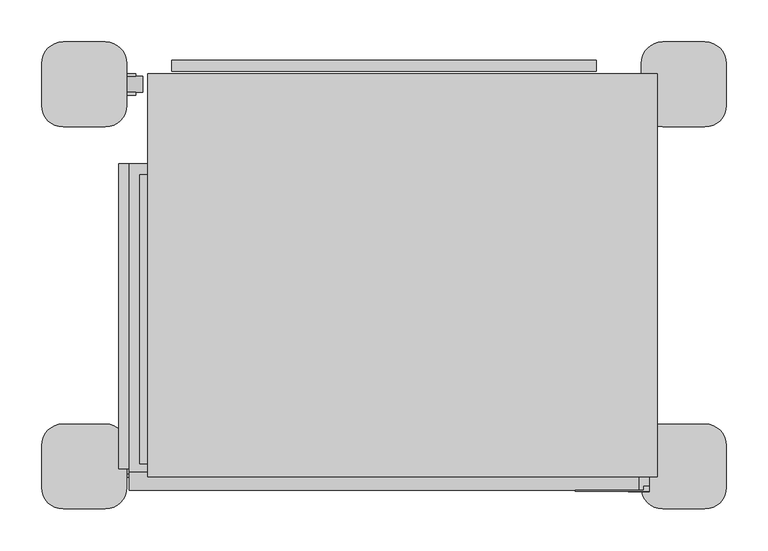
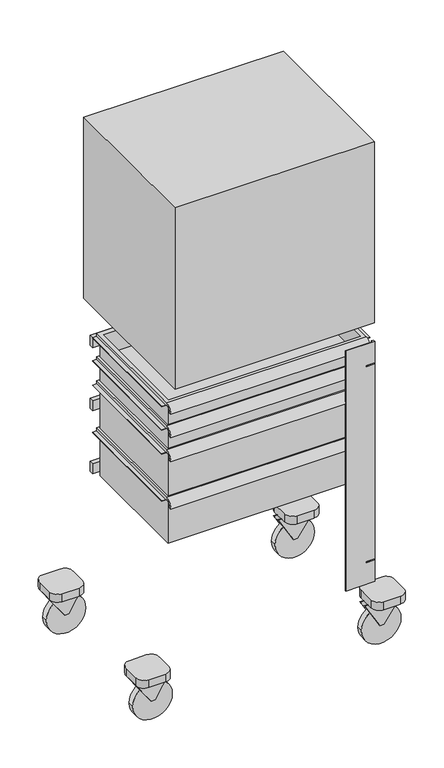
"""IFC4 building model written with IfcOpenShell, lengths in millimetres: proxy geometry, M8185 - System, Stress Exercise, w-Treadmill : M8185 - System, Stress Exercise, w-Treadmill."""

import ifcopenshell
import ifcopenshell.guid

model = None  # the IFC model being written
_history = None  # IfcOwnerHistory: only IFC2X3 demands one
_inside = {}  # id of a spatial element -> (the spatial element, [elements in it])
_under = {}  # id of a project, library or spatial element -> (it, [spatial elements below it])
_declared = {}  # id of a project -> (the project, [libraries it declares])
_typed = {}  # id of a type object -> (the type object, [elements of that type])
_made_of = {}  # id of a material, layer set ... -> (it, [elements and type objects made of it])


def new_model(schema):
    """Start an empty IFC model of exactly this schema.

    Asked for "IFC4X3", IfcOpenShell would pick the latest addendum, in which some entities
    have other attributes; the version numbers below select the first issue.
    IFC2X3 requires an IfcOwnerHistory on every rooted entity: one is made here for all.
    """
    global model, _history
    if schema == "IFC4X3":
        model = ifcopenshell.file(schema_version=(4, 3, 0, 0))
    else:
        model = ifcopenshell.file(schema=schema)
    _inside.clear()
    _under.clear()
    _declared.clear()
    _typed.clear()
    _made_of.clear()
    _history = None
    if model.schema == "IFC2X3":
        org = make("IfcOrganization", Name="unknown")
        user = make(
            "IfcPersonAndOrganization",
            ThePerson=make("IfcPerson", FamilyName="unknown"),
            TheOrganization=org,
        )
        app = make(
            "IfcApplication",
            ApplicationDeveloper=org,
            Version="unknown",
            ApplicationFullName="unknown",
            ApplicationIdentifier="unknown",
        )
        _history = make(
            "IfcOwnerHistory",
            OwningUser=user,
            OwningApplication=app,
            ChangeAction="ADDED",
            CreationDate=0,
        )
    return model


def make(cls, **values):
    """One entity of the class cls with the attributes given. An attribute that is None is left unset."""
    return model.create_entity(
        cls, **{name: value for name, value in values.items() if value is not None}
    )


def rooted(cls, **values):
    """An entity with a GlobalId (a new one), such as an element, a storey or a relation."""
    return make(cls, GlobalId=ifcopenshell.guid.new(), OwnerHistory=_history, **values)


def si_unit(unit_type, name, prefix=None):
    """IfcSIUnit, for example si_unit("LENGTHUNIT", "METRE", prefix="MILLI")."""
    return make("IfcSIUnit", UnitType=unit_type, Prefix=prefix, Name=name)


def assignment(units):
    """IfcUnitAssignment: the units of a project."""
    return None if units is None else make("IfcUnitAssignment", Units=units)


def point(xyz):
    """IfcCartesianPoint."""
    return None if xyz is None else make("IfcCartesianPoint", Coordinates=xyz)


def direction(xyz):
    """IfcDirection."""
    return None if xyz is None else make("IfcDirection", DirectionRatios=xyz)


def frame(location, z_axis=None, x_axis=None):
    """IfcAxis2Placement3D, a coordinate frame: its origin and axes. An axis left out is left unset."""
    return make(
        "IfcAxis2Placement3D",
        Location=point(location),
        Axis=direction(z_axis),
        RefDirection=direction(x_axis),
    )


def frame_2d(location, x_axis=None):
    """IfcAxis2Placement2D, a coordinate frame in the plane: its origin and x axis."""
    return make(
        "IfcAxis2Placement2D", Location=point(location), RefDirection=direction(x_axis)
    )


def origin():
    """The frame at (0, 0, 0) with its axes left unset."""
    return frame((0.0, 0.0, 0.0))


def place(relative_to, where):
    """IfcLocalPlacement: puts the frame where relative to a parent placement (None: the world)."""
    return make(
        "IfcLocalPlacement", PlacementRelTo=relative_to, RelativePlacement=where
    )


def context(
    kind, dimensions, precision=None, world=None, true_north=None, identifier=None
):
    """IfcGeometricRepresentationContext, for example the 3D "Model" context."""
    return make(
        "IfcGeometricRepresentationContext",
        ContextIdentifier=identifier,
        ContextType=kind,
        CoordinateSpaceDimension=dimensions,
        Precision=precision,
        WorldCoordinateSystem=world,
        TrueNorth=true_north,
    )


def project(units=None, contexts=None):
    """IfcProject with its units and contexts."""
    return rooted(
        "IfcProject",
        Name="project",
        RepresentationContexts=contexts,
        UnitsInContext=assignment(units),
    )


def spatial(cls, under=None, at=None, **own):
    """A site, building, storey or space (cls), placed at a placement, below another one or the project."""
    s = rooted(cls, ObjectPlacement=at, **own)
    if under is not None:
        _under.setdefault(under.id(), (under, []))[1].append(s)
    return s


def polyline(points):
    """IfcPolyline through the points."""
    return make("IfcPolyline", Points=[point(p) for p in points])


def circle_curve(where, radius):
    """IfcCircle in the frame where."""
    return make("IfcCircle", Position=where, Radius=radius)


def trimmed(basis, trim1, trim2, sense, master):
    """IfcTrimmedCurve: the piece of a basis curve between two trims."""
    return make(
        "IfcTrimmedCurve",
        BasisCurve=basis,
        Trim1=trim1,
        Trim2=trim2,
        SenseAgreement=sense,
        MasterRepresentation=master,
    )


def segment(curve, same_sense, transition):
    """IfcCompositeCurveSegment."""
    return make(
        "IfcCompositeCurveSegment",
        Transition=transition,
        SameSense=same_sense,
        ParentCurve=curve,
    )


def composite_curve(segments, self_intersect=None):
    """IfcCompositeCurve: segments joined end to end."""
    return make("IfcCompositeCurve", Segments=segments, SelfIntersect=self_intersect)


def outline(outer, holes=None, kind="AREA"):
    """IfcArbitraryClosedProfileDef: a profile drawn as a closed curve; with holes, ...WithVoids."""
    if holes is None:
        return make("IfcArbitraryClosedProfileDef", ProfileType=kind, OuterCurve=outer)
    return make(
        "IfcArbitraryProfileDefWithVoids",
        ProfileType=kind,
        OuterCurve=outer,
        InnerCurves=holes,
    )


def extrude(swept, where, along, depth):
    """IfcExtrudedAreaSolid: the profile swept, set in the frame where, extruded along a direction by depth."""
    return make(
        "IfcExtrudedAreaSolid",
        SweptArea=swept,
        Position=where,
        ExtrudedDirection=direction(along),
        Depth=depth,
    )


def faces_of(points, faces, orient=None, outer=None):
    """IfcFace entities. A face is a list of loops; a loop is a list of indices into points, from 0.

    orient and outer hold one flag for each loop. By default every Orientation is true, the
    first loop of a face is its IfcFaceOuterBound and the others are IfcFaceBound.
    """
    made = []
    for i, loops in enumerate(faces):
        bounds = []
        for j, loop in enumerate(loops):
            is_outer = j == 0 if outer is None else outer[i][j]
            bounds.append(
                make(
                    "IfcFaceOuterBound" if is_outer else "IfcFaceBound",
                    Bound=make("IfcPolyLoop", Polygon=[points[k] for k in loop]),
                    Orientation=True if orient is None else orient[i][j],
                )
            )
        made.append(make("IfcFace", Bounds=bounds))
    return made


def faceted_brep(points, faces, orient=None, outer=None, voids=None):
    """IfcFacetedBrep: a solid bounded by flat faces; with voids (closed shells), ...WithVoids."""
    shared = [point(p) for p in points]
    hull = make("IfcClosedShell", CfsFaces=faces_of(shared, faces, orient, outer))
    if voids is None:
        return make("IfcFacetedBrep", Outer=hull)
    return make(
        "IfcFacetedBrepWithVoids",
        Outer=hull,
        Voids=[
            make(cls, CfsFaces=faces_of(shared, fs, o, b)) for cls, fs, o, b in voids
        ],
    )


def shape(context_of_items, identifier, shape_type, items):
    """IfcShapeRepresentation: the items that make up one representation, for example the "Body"."""
    return make(
        "IfcShapeRepresentation",
        ContextOfItems=context_of_items,
        RepresentationIdentifier=identifier,
        RepresentationType=shape_type,
        Items=items,
    )


def source(mapping_origin, context_of_items, identifier, shape_type, items):
    """IfcRepresentationMap: a shape defined once, which mapped items show again and again."""
    return make(
        "IfcRepresentationMap",
        MappingOrigin=mapping_origin,
        MappedRepresentation=shape(context_of_items, identifier, shape_type, items),
    )


def transform(
    local_origin,
    x_axis=None,
    y_axis=None,
    z_axis=None,
    scale=None,
    scale2=None,
    scale3=None,
    uniform=True,
):
    """IfcCartesianTransformationOperator3D, or its non-uniform kind. x_axis, y_axis, z_axis: its Axis1, 2, 3."""
    if uniform:
        return make(
            "IfcCartesianTransformationOperator3D",
            Axis1=direction(x_axis),
            Axis2=direction(y_axis),
            LocalOrigin=point(local_origin),
            Scale=scale,
            Axis3=direction(z_axis),
        )
    return make(
        "IfcCartesianTransformationOperator3DnonUniform",
        Axis1=direction(x_axis),
        Axis2=direction(y_axis),
        LocalOrigin=point(local_origin),
        Scale=scale,
        Axis3=direction(z_axis),
        Scale2=scale2,
        Scale3=scale3,
    )


def mapped(mapping_source, mapping_target):
    """IfcMappedItem: shows the shape of a source again, moved by a transform."""
    return make(
        "IfcMappedItem", MappingSource=mapping_source, MappingTarget=mapping_target
    )


def made_of(thing, what):
    """Note that an element or type object is made of a material, layer set ...; save() writes the relation."""
    if what is not None:
        _made_of.setdefault(what.id(), (what, []))[1].append(thing)
    return thing


def element(
    cls,
    number,
    at=None,
    inside=None,
    cuts=None,
    type_object=None,
    material=None,
    context=None,
    identifier="Body",
    shape_type=None,
    held_by="IfcProductDefinitionShape",
    body=None,
    shapes=None,
    **own,
):
    """One element of the class cls, such as IfcWall. Its Tag is "e" and its number.

    at: its placement. inside: the storey or other place that contains it. cuts: it is an
    opening in that element (IfcRelVoidsElement). A single representation is given by context,
    identifier, shape_type and body (its items); several are given by shapes. held_by: the class
    of the entity that holds the representations. save() writes the other relations.
    """
    e = rooted(cls, Tag="e%d" % number, ObjectPlacement=at, **own)
    if body is not None:
        shapes = [shape(context, identifier, shape_type, body)]
    if shapes is not None:
        e.Representation = make(held_by, Representations=shapes)
    if inside is not None:
        _inside.setdefault(inside.id(), (inside, []))[1].append(e)
    if cuts is not None:
        rooted(
            "IfcRelVoidsElement", RelatingBuildingElement=cuts, RelatedOpeningElement=e
        )
    if type_object is not None:
        _typed.setdefault(type_object.id(), (type_object, []))[1].append(e)
    return made_of(e, material)


def aggregate(whole, parts):
    """IfcRelAggregates: a whole, such as a stair, and the parts it consists of."""
    return rooted("IfcRelAggregates", RelatingObject=whole, RelatedObjects=parts)


def save(model, path):
    """Write the relations noted so far, then the file.

    IfcRelAggregates (storeys below a building ...), IfcRelContainedInSpatialStructure (elements
    in a storey), IfcRelDefinesByType, IfcRelAssociatesMaterial and IfcRelDeclares: one each for
    every whole, place, type object, material and project.
    """
    for whole, parts in _under.values():
        aggregate(whole, parts)
    for where, things in _inside.values():
        rooted(
            "IfcRelContainedInSpatialStructure",
            RelatedElements=things,
            RelatingStructure=where,
        )
    for kind, things in _typed.values():
        rooted("IfcRelDefinesByType", RelatedObjects=things, RelatingType=kind)
    for what, things in _made_of.values():
        rooted("IfcRelAssociatesMaterial", RelatedObjects=things, RelatingMaterial=what)
    for by, libraries in _declared.values():
        rooted("IfcRelDeclares", RelatingContext=by, RelatedDefinitions=libraries)
    model.write(path)


def plane_surface(at):
    """IfcPlane: the flat surface through the origin of the frame at, square to its z axis."""
    return make("IfcPlane", Position=at)


def cylinder_surface(at, radius):
    """IfcCylindricalSurface: all points at the distance radius from the z axis of the frame at."""
    return make("IfcCylindricalSurface", Position=at, Radius=radius)


def revolved_surface(curve, axis_point, axis_direction):
    """IfcSurfaceOfRevolution: the curve turned about the line through axis_point along axis_direction."""
    return make(
        "IfcSurfaceOfRevolution",
        SweptCurve=make("IfcArbitraryOpenProfileDef", ProfileType="CURVE", Curve=curve),
        AxisPosition=make("IfcAxis1Placement", Location=point(axis_point), Axis=direction(axis_direction)),
    )


def advanced_brep(points, edges, surfaces, faces):
    """IfcAdvancedBrep: a solid bounded by faces that lie on surfaces and meet in shared edges.

    An edge is (start, end): straight between two places in points (the first is 0);
    or (start, end, curve); or (start, end, curve, False) where it runs against its curve.
    A face is (place in surfaces, loops), or (place, loops, False) where it looks against
    its surface's normal. A loop lists edges by number (the first is 1), with a minus sign
    where the edge is run from its end to its start. The first loop is the outer one.
    """
    corners = [point(p) for p in points]
    vertices = [make("IfcVertexPoint", VertexGeometry=c) for c in corners]
    made = []
    for start, end, *more in edges:
        made.append(
            make(
                "IfcEdgeCurve",
                EdgeStart=vertices[start],
                EdgeEnd=vertices[end],
                EdgeGeometry=more[0] if more else make("IfcPolyline", Points=[corners[start], corners[end]]),
                SameSense=more[1] if len(more) > 1 else True,
            )
        )
    hull = []
    for where, loops, *sense in faces:
        bounds = []
        for j, loop in enumerate(loops):
            ring = [make("IfcOrientedEdge", EdgeElement=made[abs(k) - 1], Orientation=k > 0) for k in loop]
            bounds.append(
                make(
                    "IfcFaceOuterBound" if j == 0 else "IfcFaceBound",
                    Bound=make("IfcEdgeLoop", EdgeList=ring),
                    Orientation=True,
                )
            )
        hull.append(make("IfcAdvancedFace", Bounds=bounds, FaceSurface=surfaces[where], SameSense=sense[0] if sense else True))
    return make("IfcAdvancedBrep", Outer=make("IfcClosedShell", CfsFaces=hull))


def specialty_equipment_8ec998c3(model_context):
    return source(origin(), model_context, "Body", "SolidModel", [
        faceted_brep([(-177.3747223, 933.9418342, 1473.2), (-659.9747223, 933.9418342, 1473.2), (-659.9747223, 883.3104531, 1473.2), (-177.3747223, 883.3104531, 1473.2), (-177.3747223, 933.9418342, 1193.8), (-177.3747223, 883.3104531, 1193.8), (-659.9747223, 883.3104531, 1193.8), (-659.9747223, 933.9418342, 1193.8), (-647.2747223, 883.3104531, 1460.5), (-190.0747223, 883.3104531, 1460.5), (-190.0747223, 883.3104531, 1206.5), (-647.2747223, 883.3104531, 1206.5), (-190.0747223, 888.0966556, 1460.5), (-647.2747223, 888.0966556, 1460.5), (-190.0747223, 888.0966556, 1206.5), (-647.2747223, 888.0966556, 1206.5)], [[[0, 1, 2, 3]], [[4, 5, 6, 7]], [[1, 0, 4, 7]], [[2, 1, 7, 6]], [[3, 2, 6, 5], [8, 9, 10, 11]], [[0, 3, 5, 4]], [[12, 9, 8, 13]], [[14, 15, 11, 10]], [[12, 13, 15, 14]], [[13, 8, 11, 15]], [[9, 12, 14, 10]]]),
        extrude(outline(polyline([(584.7761437, 1054.1), (737.1761437, 1066.8), (737.1761437, 1041.4), (584.7761437, 1041.4), (584.7761437, 1054.1)])), frame((-659.9747223, 0.0, 0.0), z_axis=(1.0, 0.0, 0.0), x_axis=(0.0, 1.0, 0.0)), (0.0, 0.0, 1.0), 482.6),
        faceted_brep([(-271.4528828, 800.6761437, 1066.8), (-271.4528828, 800.6761437, 1041.4), (-271.4528828, 1016.5761437, 1041.4), (-271.4528828, 1016.5761437, 1066.8), (-565.8965618, 1016.5761437, 1066.8), (-565.8965618, 1016.5761437, 1041.4), (-565.8965618, 800.6761437, 1041.4), (-565.8965618, 800.6761437, 1066.8), (-381.7061537, 997.4418342, 1073.15), (-381.7061537, 997.4418342, 1066.8), (-455.6432909, 997.4418342, 1066.8), (-455.6432909, 997.4418342, 1073.15), (-381.7061537, 997.4418342, 1333.5), (-455.6432909, 997.4418342, 1333.5), (-381.7061537, 933.9418342, 1333.5), (-455.6432909, 933.9418342, 1333.5), (-381.7061537, 933.9418342, 1282.7), (-455.6432909, 933.9418342, 1282.7), (-381.7061537, 972.0418342, 1282.7), (-455.6432909, 972.0418342, 1282.7), (-381.7061537, 972.0418342, 1066.8), (-455.6432909, 972.0418342, 1066.8)], [[[0, 1, 2, 3]], [[4, 5, 6, 7]], [[8, 9, 10, 11]], [[12, 8, 11, 13]], [[14, 12, 13, 15]], [[16, 14, 15, 17]], [[18, 16, 17, 19]], [[20, 18, 19, 21]], [[0, 3, 4, 7], [9, 20, 21, 10]], [[1, 0, 7, 6]], [[2, 1, 6, 5]], [[3, 2, 5, 4]], [[20, 9, 8, 12, 14, 16, 18]], [[10, 21, 19, 17, 15, 13, 11]]]),
        extrude(outline(polyline([(-113.8747223, 1041.9761437), (-113.8747223, 559.3761437), (-723.4747223, 559.3761437), (-723.4747223, 1041.9761437), (-113.8747223, 1041.9761437)])), frame((0.0, 0.0, 1041.4), z_axis=(0.0, 0.0, 1.0), x_axis=(1.0, 0.0, 0.0)), (0.0, 0.0, 1.0), 584.2),
        extrude(outline(polyline([(-186.8997223, 1057.8511437), (-186.8997223, 1045.1511437), (-694.8997223, 1045.1511437), (-694.8997223, 1057.8511437), (-186.8997223, 1057.8511437)])), frame((0.0, 0.0, 464.30692), z_axis=(0.0, 0.0, 1.0), x_axis=(1.0, 0.0, 0.0)), (0.0, 0.0, 1.0), 31.75),
        extrude(outline(polyline([(-186.8997223, 1057.8511437), (-186.8997223, 1045.1511437), (-694.8997223, 1045.1511437), (-694.8997223, 1057.8511437), (-186.8997223, 1057.8511437)])), frame((0.0, 0.0, 667.50692), z_axis=(0.0, 0.0, 1.0), x_axis=(1.0, 0.0, 0.0)), (0.0, 0.0, 1.0), 31.75),
        extrude(outline(polyline([(-186.8997223, 1057.8511437), (-186.8997223, 1045.1511437), (-694.8997223, 1045.1511437), (-694.8997223, 1057.8511437), (-186.8997223, 1057.8511437)])), frame((0.0, 0.0, 870.70692), z_axis=(0.0, 0.0, 1.0), x_axis=(1.0, 0.0, 0.0)), (0.0, 0.0, 1.0), 31.75),
        advanced_brep(
        [(-739.3497223, 569.0376764, 696.8915302), (-142.4497223, 569.0376764, 696.8915302), (-142.4497223, 569.0376764, 838.1917302), (-123.3997223, 569.0376764, 838.1917302), (-123.3997223, 569.0376764, 839.7792302), (-136.0997223, 569.0376764, 839.7792302), (-136.0997223, 569.0376764, 842.9415302), (-745.6997223, 569.0376764, 842.9415302), (-745.6997223, 569.0376764, 839.7792302), (-758.3997223, 569.0376764, 839.7792302), (-758.3997223, 569.0376764, 838.1917302), (-739.3497223, 569.0376764, 838.1917302), (-142.4497223, 927.8126764, 696.8915302), (-739.3497223, 927.8126764, 696.8915302), (-739.3497223, 927.8126764, 838.1917302), (-142.4497223, 927.8126764, 838.1917302), (-136.0997223, 565.7634577, 849.2915302), (-136.0997223, 934.1626764, 849.2915302), (-745.6997223, 934.1626764, 849.2915302), (-745.6997223, 565.7634577, 849.2915302), (-148.7997223, 575.3876764, 849.2915302), (-732.9997223, 575.3876764, 849.2915302), (-732.9997223, 920.8276764, 849.2915302), (-148.7997223, 920.8276764, 849.2915302), (-136.0997223, 543.6376764, 824.6484502), (-136.0997223, 550.0395136, 824.6484502), (-136.0997223, 565.7634577, 842.9415302), (-136.0997223, 934.1626764, 839.7792302), (-745.6997223, 565.7634577, 842.9415302), (-745.6997223, 550.0395136, 824.6484502), (-745.6997223, 543.6376764, 824.6484502), (-745.6997223, 934.1626764, 839.7792302), (-123.3997223, 934.1626764, 838.1917302), (-758.3997223, 934.1626764, 838.1917302), (-123.3997223, 934.1626764, 839.7792302), (-758.3997223, 934.1626764, 839.7792302), (-732.9997223, 575.3876764, 706.4165302), (-148.7997223, 575.3876764, 706.4165302), (-148.7997223, 920.8276764, 706.4165302), (-732.9997223, 920.8276764, 706.4165302)],
        [
            (0, 1),
            (1, 2),
            (2, 3),
            (3, 4),
            (4, 5),
            (5, 6),
            (6, 7),
            (7, 8),
            (8, 9),
            (9, 10),
            (10, 11),
            (11, 0),
            (12, 13),
            (13, 14),
            (14, 15),
            (15, 12),
            (0, 13),
            (12, 1),
            (15, 2),
            (16, 17),
            (17, 18),
            (18, 19),
            (19, 16),
            (20, 21),
            (21, 22),
            (22, 23),
            (23, 20),
            (11, 14),
            (16, 24, circle_curve(frame((-136.0997223, 565.7634577, 827.0371775), z_axis=(1.0, 0.0, 0.0), x_axis=(0.0, 1.0, 0.0)), 22.2543527)),
            (24, 25),
            (25, 26, circle_curve(frame((-136.0997223, 565.7634577, 827.0371775), z_axis=(-1.0, 0.0, 0.0), x_axis=(0.0, 1.0, 0.0)), 15.9043527)),
            (26, 6),
            (5, 27),
            (27, 17),
            (7, 28),
            (28, 29, circle_curve(frame((-745.6997223, 565.7634577, 827.0371775), z_axis=(1.0, 0.0, 0.0), x_axis=(0.0, 1.0, 0.0)), 15.9043527)),
            (29, 30),
            (30, 19, circle_curve(frame((-745.6997223, 565.7634577, 827.0371775), z_axis=(-1.0, 0.0, 0.0), x_axis=(0.0, 1.0, 0.0)), 22.2543527)),
            (18, 31),
            (31, 8),
            (30, 24),
            (29, 25),
            (28, 26),
            (32, 3),
            (10, 33),
            (33, 32),
            (27, 34),
            (34, 32),
            (33, 35),
            (35, 31),
            (36, 37),
            (37, 38),
            (38, 39),
            (39, 36),
            (36, 21),
            (20, 37),
            (23, 38),
            (22, 39),
            (9, 35),
            (4, 34),
        ],
        [
            plane_surface(frame((-142.4497223, 569.0376764, 696.8915302), z_axis=(0.0, -1.0, 0.0), x_axis=(1.0, 0.0, 0.0))),
            plane_surface(frame((-142.4497223, 927.8126764, 696.8915302), z_axis=(0.0, 1.0, 0.0), x_axis=(-1.0, 0.0, 0.0))),
            plane_surface(frame((-739.3497223, 569.0376764, 696.8915302), z_axis=(0.0, 0.0, -1.0), x_axis=(0.0, 1.0, 0.0))),
            plane_surface(frame((-142.4497223, 569.0376764, 696.8915302), z_axis=(1.0, 0.0, 0.0), x_axis=(0.0, 1.0, 0.0))),
            plane_surface(frame((-142.4497223, 569.0376764, 849.2915302), z_axis=(0.0, 0.0, 1.0), x_axis=(0.0, 1.0, 0.0))),
            plane_surface(frame((-739.3497223, 569.0376764, 849.2915302), z_axis=(-1.0, 0.0, 0.0), x_axis=(0.0, 1.0, 0.0))),
            plane_surface(frame((-136.0997223, 934.1626764, 849.2915302), z_axis=(1.0, 0.0, 0.0), x_axis=(0.0, -1.0, 0.0))),
            plane_surface(frame((-745.6997223, 934.1626764, 849.2915302), z_axis=(-1.0, 0.0, 0.0), x_axis=(0.0, 1.0, 0.0))),
            cylinder_surface(frame((-745.6997223, 565.7634577, 827.0371775), z_axis=(1.0, 0.0, 0.0), x_axis=(0.0, 1.0, 0.0)), 22.2543527),
            plane_surface(frame((-136.0997223, 543.6376764, 824.6484502), z_axis=(0.0, 0.0, -1.0), x_axis=(-1.0, 0.0, 0.0))),
            revolved_surface(polyline([(-745.6997223, 581.6678104, 827.0371775), (-136.09972230000005, 581.6678104, 827.0371775)]), (-745.6997223, 565.7634577, 827.0371775), (-1.0, 0.0, 0.0)),
            plane_surface(frame((-136.0997223, 565.7634577, 842.9415302), z_axis=(0.0, -1.0696897912904252e-12, -1.0), x_axis=(-1.0, 0.0, 0.0))),
            plane_surface(frame((-136.0997223, 569.0376764, 838.1917302), z_axis=(0.0, 0.0, -1.0), x_axis=(-1.0, 0.0, 0.0))),
            plane_surface(frame((-136.0997223, 934.1626764, 838.1917302), z_axis=(0.0, 1.0, 0.0), x_axis=(-1.0, 0.0, 0.0))),
            plane_surface(frame((-148.7997223, 575.3876764, 706.4165302), z_axis=(0.0, 0.0, 1.0), x_axis=(-1.0, 0.0, 0.0))),
            plane_surface(frame((-732.9997223, 575.3876764, 849.2915302), z_axis=(0.0, 1.0, 0.0), x_axis=(0.0, 0.0, -1.0))),
            plane_surface(frame((-148.7997223, 575.3876764, 849.2915302), z_axis=(-1.0, 0.0, 0.0), x_axis=(0.0, 0.0, -1.0))),
            plane_surface(frame((-148.7997223, 920.8276764, 849.2915302), z_axis=(0.0, -1.0, 0.0), x_axis=(0.0, 0.0, -1.0))),
            plane_surface(frame((-732.9997223, 920.8276764, 849.2915302), z_axis=(1.0, 0.0, 0.0), x_axis=(0.0, 0.0, -1.0))),
            plane_surface(frame((-758.3997223, 934.1626764, 838.1917302), z_axis=(-1.0, 0.0, 0.0), x_axis=(0.0, -1.0, 0.0))),
            plane_surface(frame((-758.3997223, 934.1626764, 839.7792302), z_axis=(0.0, 0.0, 1.0), x_axis=(0.0, -1.0, 0.0))),
            plane_surface(frame((-136.0997223, 934.1626764, 839.7792302), z_axis=(0.0, 0.0, 1.0), x_axis=(0.0, -1.0, 0.0))),
            plane_surface(frame((-123.3997223, 934.1626764, 839.7792302), z_axis=(1.0, 0.0, 0.0), x_axis=(0.0, -1.0, 0.0))),
        ],
        [
            (0, [[1, 2, 3, 4, 5, 6, 7, 8, 9, 10, 11, 12]]),
            (1, [[13, 14, 15, 16]]),
            (2, [[-1, 17, -13, 18]]),
            (3, [[-18, -16, 19, -2]]),
            (4, [[20, 21, 22, 23], [24, 25, 26, 27]]),
            (5, [[-17, -12, 28, -14]]),
            (6, [[-20, 29, 30, 31, 32, -6, 33, 34]]),
            (7, [[35, 36, 37, 38, -22, 39, 40, -8]]),
            (8, [[-29, -23, -38, 41]]),
            (9, [[-30, -41, -37, 42]]),
            (10, [[-31, -42, -36, 43]]),
            (11, [[-32, -43, -35, -7]]),
            (12, [[44, -3, -19, -15, -28, -11, 45, 46]]),
            (13, [[-21, -34, 47, 48, -46, 49, 50, -39]]),
            (14, [[51, 52, 53, 54]]),
            (15, [[-51, 55, -24, 56]]),
            (16, [[-52, -56, -27, 57]]),
            (17, [[-53, -57, -26, 58]]),
            (18, [[-54, -58, -25, -55]]),
            (19, [[-49, -45, -10, 59]]),
            (20, [[-50, -59, -9, -40]]),
            (21, [[-47, -33, -5, 60]]),
            (22, [[-48, -60, -4, -44]]),
        ],
    ),
        extrude(outline(polyline([(-123.3997223, 564.2751764), (-123.3997223, 542.0501764), (-148.7997223, 542.0501764), (-148.7997223, 564.2751764), (-123.3997223, 564.2751764)])), frame((0.0, 0.0, 923.417), z_axis=(0.0, 0.0, 1.0), x_axis=(1.0, 0.0, 0.0)), (0.0, 0.0, 1.0), 3.175),
        extrude(outline(polyline([(-123.3997223, 564.2751764), (-123.3997223, 542.0501764), (-148.7997223, 542.0501764), (-148.7997223, 564.2751764), (-123.3997223, 564.2751764)])), frame((0.0, 0.0, 291.592), z_axis=(0.0, 0.0, 1.0), x_axis=(1.0, 0.0, 0.0)), (0.0, 0.0, 1.0), 3.175),
        extrude(outline(polyline([(-123.3997223, 542.0501764), (-212.2997223, 542.0501764), (-212.2997223, 543.6376764), (-129.7497223, 543.6376764), (-129.7497223, 548.4001764), (-123.3997223, 548.4001764), (-123.3997223, 542.0501764)])), frame((0.0, 0.0, 221.742), z_axis=(0.0, 0.0, 1.0), x_axis=(1.0, 0.0, 0.0)), (0.0, 0.0, 1.0), 774.7),
        advanced_brep(
        [(-739.3497223, 569.0376764, 544.4915302), (-142.4497223, 569.0376764, 544.4915302), (-142.4497223, 569.0376764, 685.7917302), (-123.3997223, 569.0376764, 685.7917302), (-123.3997223, 569.0376764, 687.3792302), (-136.0997223, 569.0376764, 687.3792302), (-136.0997223, 569.0376764, 690.5415302), (-745.6997223, 569.0376764, 690.5415302), (-745.6997223, 569.0376764, 687.3792302), (-758.3997223, 569.0376764, 687.3792302), (-758.3997223, 569.0376764, 685.7917302), (-739.3497223, 569.0376764, 685.7917302), (-142.4497223, 927.8126764, 544.4915302), (-739.3497223, 927.8126764, 544.4915302), (-739.3497223, 927.8126764, 685.7917302), (-142.4497223, 927.8126764, 685.7917302), (-136.0997223, 565.7634577, 696.8915302), (-136.0997223, 934.1626764, 696.8915302), (-745.6997223, 934.1626764, 696.8915302), (-745.6997223, 565.7634577, 696.8915302), (-148.7997223, 575.3876764, 696.8915302), (-732.9997223, 575.3876764, 696.8915302), (-732.9997223, 920.8276764, 696.8915302), (-148.7997223, 920.8276764, 696.8915302), (-136.0997223, 543.6376764, 672.2484502), (-136.0997223, 550.0395136, 672.2484502), (-136.0997223, 565.7634577, 690.5415302), (-136.0997223, 934.1626764, 687.3792302), (-745.6997223, 565.7634577, 690.5415302), (-745.6997223, 550.0395136, 672.2484502), (-745.6997223, 543.6376764, 672.2484502), (-745.6997223, 934.1626764, 687.3792302), (-123.3997223, 934.1626764, 685.7917302), (-758.3997223, 934.1626764, 685.7917302), (-123.3997223, 934.1626764, 687.3792302), (-758.3997223, 934.1626764, 687.3792302), (-732.9997223, 575.3876764, 554.0165302), (-148.7997223, 575.3876764, 554.0165302), (-148.7997223, 920.8276764, 554.0165302), (-732.9997223, 920.8276764, 554.0165302)],
        [
            (0, 1),
            (1, 2),
            (2, 3),
            (3, 4),
            (4, 5),
            (5, 6),
            (6, 7),
            (7, 8),
            (8, 9),
            (9, 10),
            (10, 11),
            (11, 0),
            (12, 13),
            (13, 14),
            (14, 15),
            (15, 12),
            (0, 13),
            (12, 1),
            (15, 2),
            (16, 17),
            (17, 18),
            (18, 19),
            (19, 16),
            (20, 21),
            (21, 22),
            (22, 23),
            (23, 20),
            (11, 14),
            (16, 24, circle_curve(frame((-136.0997223, 565.7634577, 674.6371775), z_axis=(1.0, 0.0, 0.0), x_axis=(0.0, 1.0, 0.0)), 22.2543527)),
            (24, 25),
            (25, 26, circle_curve(frame((-136.0997223, 565.7634577, 674.6371775), z_axis=(-1.0, 0.0, 0.0), x_axis=(0.0, 1.0, 0.0)), 15.9043527)),
            (26, 6),
            (5, 27),
            (27, 17),
            (7, 28),
            (28, 29, circle_curve(frame((-745.6997223, 565.7634577, 674.6371775), z_axis=(1.0, 0.0, 0.0), x_axis=(0.0, 1.0, 0.0)), 15.9043527)),
            (29, 30),
            (30, 19, circle_curve(frame((-745.6997223, 565.7634577, 674.6371775), z_axis=(-1.0, 0.0, 0.0), x_axis=(0.0, 1.0, 0.0)), 22.2543527)),
            (18, 31),
            (31, 8),
            (30, 24),
            (29, 25),
            (28, 26),
            (32, 3),
            (10, 33),
            (33, 32),
            (27, 34),
            (34, 32),
            (33, 35),
            (35, 31),
            (36, 37),
            (37, 38),
            (38, 39),
            (39, 36),
            (36, 21),
            (20, 37),
            (23, 38),
            (22, 39),
            (9, 35),
            (4, 34),
        ],
        [
            plane_surface(frame((-142.4497223, 569.0376764, 544.4915302), z_axis=(0.0, -1.0, 0.0), x_axis=(1.0, 0.0, 0.0))),
            plane_surface(frame((-142.4497223, 927.8126764, 544.4915302), z_axis=(0.0, 1.0, 0.0), x_axis=(-1.0, 0.0, 0.0))),
            plane_surface(frame((-739.3497223, 569.0376764, 544.4915302), z_axis=(0.0, 0.0, -1.0), x_axis=(0.0, 1.0, 0.0))),
            plane_surface(frame((-142.4497223, 569.0376764, 544.4915302), z_axis=(1.0, 0.0, 0.0), x_axis=(0.0, 1.0, 0.0))),
            plane_surface(frame((-142.4497223, 569.0376764, 696.8915302), z_axis=(0.0, 0.0, 1.0), x_axis=(0.0, 1.0, 0.0))),
            plane_surface(frame((-739.3497223, 569.0376764, 696.8915302), z_axis=(-1.0, 0.0, 0.0), x_axis=(0.0, 1.0, 0.0))),
            plane_surface(frame((-136.0997223, 934.1626764, 696.8915302), z_axis=(1.0, 0.0, 0.0), x_axis=(0.0, -1.0, 0.0))),
            plane_surface(frame((-745.6997223, 934.1626764, 696.8915302), z_axis=(-1.0, 0.0, 0.0), x_axis=(0.0, 1.0, 0.0))),
            cylinder_surface(frame((-745.6997223, 565.7634577, 674.6371775), z_axis=(1.0, 0.0, 0.0), x_axis=(0.0, 1.0, 0.0)), 22.2543527),
            plane_surface(frame((-136.0997223, 543.6376764, 672.2484502), z_axis=(0.0, 0.0, -1.0), x_axis=(-1.0, 0.0, 0.0))),
            revolved_surface(polyline([(-745.6997223, 581.6678104, 674.6371775), (-136.09972230000005, 581.6678104, 674.6371775)]), (-745.6997223, 565.7634577, 674.6371775), (-1.0, 0.0, 0.0)),
            plane_surface(frame((-136.0997223, 565.7634577, 690.5415302), z_axis=(0.0, -1.0696897912904252e-12, -1.0), x_axis=(-1.0, 0.0, 0.0))),
            plane_surface(frame((-136.0997223, 569.0376764, 685.7917302), z_axis=(0.0, 0.0, -1.0), x_axis=(-1.0, 0.0, 0.0))),
            plane_surface(frame((-136.0997223, 934.1626764, 685.7917302), z_axis=(0.0, 1.0, 0.0), x_axis=(-1.0, 0.0, 0.0))),
            plane_surface(frame((-148.7997223, 575.3876764, 554.0165302), z_axis=(0.0, 0.0, 1.0), x_axis=(-1.0, 0.0, 0.0))),
            plane_surface(frame((-732.9997223, 575.3876764, 696.8915302), z_axis=(0.0, 1.0, 0.0), x_axis=(0.0, 0.0, -1.0))),
            plane_surface(frame((-148.7997223, 575.3876764, 696.8915302), z_axis=(-1.0, 0.0, 0.0), x_axis=(0.0, 0.0, -1.0))),
            plane_surface(frame((-148.7997223, 920.8276764, 696.8915302), z_axis=(0.0, -1.0, 0.0), x_axis=(0.0, 0.0, -1.0))),
            plane_surface(frame((-732.9997223, 920.8276764, 696.8915302), z_axis=(1.0, 0.0, 0.0), x_axis=(0.0, 0.0, -1.0))),
            plane_surface(frame((-758.3997223, 934.1626764, 685.7917302), z_axis=(-1.0, 0.0, 0.0), x_axis=(0.0, -1.0, 0.0))),
            plane_surface(frame((-758.3997223, 934.1626764, 687.3792302), z_axis=(0.0, 0.0, 1.0), x_axis=(0.0, -1.0, 0.0))),
            plane_surface(frame((-136.0997223, 934.1626764, 687.3792302), z_axis=(0.0, 0.0, 1.0), x_axis=(0.0, -1.0, 0.0))),
            plane_surface(frame((-123.3997223, 934.1626764, 687.3792302), z_axis=(1.0, 0.0, 0.0), x_axis=(0.0, -1.0, 0.0))),
        ],
        [
            (0, [[1, 2, 3, 4, 5, 6, 7, 8, 9, 10, 11, 12]]),
            (1, [[13, 14, 15, 16]]),
            (2, [[-1, 17, -13, 18]]),
            (3, [[-18, -16, 19, -2]]),
            (4, [[20, 21, 22, 23], [24, 25, 26, 27]]),
            (5, [[-17, -12, 28, -14]]),
            (6, [[-20, 29, 30, 31, 32, -6, 33, 34]]),
            (7, [[35, 36, 37, 38, -22, 39, 40, -8]]),
            (8, [[-29, -23, -38, 41]]),
            (9, [[-30, -41, -37, 42]]),
            (10, [[-31, -42, -36, 43]]),
            (11, [[-32, -43, -35, -7]]),
            (12, [[44, -3, -19, -15, -28, -11, 45, 46]]),
            (13, [[-21, -34, 47, 48, -46, 49, 50, -39]]),
            (14, [[51, 52, 53, 54]]),
            (15, [[-51, 55, -24, 56]]),
            (16, [[-52, -56, -27, 57]]),
            (17, [[-53, -57, -26, 58]]),
            (18, [[-54, -58, -25, -55]]),
            (19, [[-49, -45, -10, 59]]),
            (20, [[-50, -59, -9, -40]]),
            (21, [[-47, -33, -5, 60]]),
            (22, [[-48, -60, -4, -44]]),
        ],
    ),
        advanced_brep(
        [(-739.3497223, 569.0376764, 925.4915302), (-142.4497223, 569.0376764, 925.4915302), (-142.4497223, 569.0376764, 990.5917302), (-123.3997223, 569.0376764, 990.5917302), (-123.3997223, 569.0376764, 992.1792302), (-136.0997223, 569.0376764, 992.1792302), (-136.0997223, 569.0376764, 995.3415302), (-745.6997223, 569.0376764, 995.3415302), (-745.6997223, 569.0376764, 992.1792302), (-758.3997223, 569.0376764, 992.1792302), (-758.3997223, 569.0376764, 990.5917302), (-739.3497223, 569.0376764, 990.5917302), (-142.4497223, 927.8126764, 925.4915302), (-739.3497223, 927.8126764, 925.4915302), (-739.3497223, 927.8126764, 990.5917302), (-142.4497223, 927.8126764, 990.5917302), (-136.0997223, 565.7634577, 1001.6915302), (-136.0997223, 934.1626764, 1001.6915302), (-745.6997223, 934.1626764, 1001.6915302), (-745.6997223, 565.7634577, 1001.6915302), (-148.7997223, 575.3876764, 1001.6915302), (-732.9997223, 575.3876764, 1001.6915302), (-732.9997223, 920.8276764, 1001.6915302), (-148.7997223, 920.8276764, 1001.6915302), (-136.0997223, 543.6376764, 977.0484502), (-136.0997223, 550.0395136, 977.0484502), (-136.0997223, 565.7634577, 995.3415302), (-136.0997223, 934.1626764, 992.1792302), (-745.6997223, 565.7634577, 995.3415302), (-745.6997223, 550.0395136, 977.0484502), (-745.6997223, 543.6376764, 977.0484502), (-745.6997223, 934.1626764, 992.1792302), (-123.3997223, 934.1626764, 990.5917302), (-758.3997223, 934.1626764, 990.5917302), (-123.3997223, 934.1626764, 992.1792302), (-758.3997223, 934.1626764, 992.1792302), (-732.9997223, 575.3876764, 935.0165302), (-148.7997223, 575.3876764, 935.0165302), (-148.7997223, 920.8276764, 935.0165302), (-732.9997223, 920.8276764, 935.0165302)],
        [
            (0, 1),
            (1, 2),
            (2, 3),
            (3, 4),
            (4, 5),
            (5, 6),
            (6, 7),
            (7, 8),
            (8, 9),
            (9, 10),
            (10, 11),
            (11, 0),
            (12, 13),
            (13, 14),
            (14, 15),
            (15, 12),
            (0, 13),
            (12, 1),
            (15, 2),
            (16, 17),
            (17, 18),
            (18, 19),
            (19, 16),
            (20, 21),
            (21, 22),
            (22, 23),
            (23, 20),
            (11, 14),
            (16, 24, circle_curve(frame((-136.0997223, 565.7634577, 979.4371775), z_axis=(1.0, 0.0, 0.0), x_axis=(0.0, 1.0, 0.0)), 22.2543527)),
            (24, 25),
            (25, 26, circle_curve(frame((-136.0997223, 565.7634577, 979.4371775), z_axis=(-1.0, 0.0, 0.0), x_axis=(0.0, 1.0, 0.0)), 15.9043527)),
            (26, 6),
            (5, 27),
            (27, 17),
            (7, 28),
            (28, 29, circle_curve(frame((-745.6997223, 565.7634577, 979.4371775), z_axis=(1.0, 0.0, 0.0), x_axis=(0.0, 1.0, 0.0)), 15.9043527)),
            (29, 30),
            (30, 19, circle_curve(frame((-745.6997223, 565.7634577, 979.4371775), z_axis=(-1.0, 0.0, 0.0), x_axis=(0.0, 1.0, 0.0)), 22.2543527)),
            (18, 31),
            (31, 8),
            (30, 24),
            (29, 25),
            (28, 26),
            (32, 3),
            (10, 33),
            (33, 32),
            (27, 34),
            (34, 32),
            (33, 35),
            (35, 31),
            (36, 37),
            (37, 38),
            (38, 39),
            (39, 36),
            (36, 21),
            (20, 37),
            (23, 38),
            (22, 39),
            (9, 35),
            (4, 34),
        ],
        [
            plane_surface(frame((-142.4497223, 569.0376764, 925.4915302), z_axis=(0.0, -1.0, 0.0), x_axis=(1.0, 0.0, 0.0))),
            plane_surface(frame((-142.4497223, 927.8126764, 925.4915302), z_axis=(0.0, 1.0, 0.0), x_axis=(-1.0, 0.0, 0.0))),
            plane_surface(frame((-739.3497223, 569.0376764, 925.4915302), z_axis=(0.0, 0.0, -1.0), x_axis=(0.0, 1.0, 0.0))),
            plane_surface(frame((-142.4497223, 569.0376764, 925.4915302), z_axis=(1.0, 0.0, 0.0), x_axis=(0.0, 1.0, 0.0))),
            plane_surface(frame((-142.4497223, 569.0376764, 1001.6915302), z_axis=(0.0, 0.0, 1.0), x_axis=(0.0, 1.0, 0.0))),
            plane_surface(frame((-739.3497223, 569.0376764, 1001.6915302), z_axis=(-1.0, 0.0, 0.0), x_axis=(0.0, 1.0, 0.0))),
            plane_surface(frame((-136.0997223, 934.1626764, 1001.6915302), z_axis=(1.0, 0.0, 0.0), x_axis=(0.0, -1.0, 0.0))),
            plane_surface(frame((-745.6997223, 934.1626764, 1001.6915302), z_axis=(-1.0, 0.0, 0.0), x_axis=(0.0, 1.0, 0.0))),
            cylinder_surface(frame((-745.6997223, 565.7634577, 979.4371775), z_axis=(1.0, 0.0, 0.0), x_axis=(0.0, 1.0, 0.0)), 22.2543527),
            plane_surface(frame((-136.0997223, 543.6376764, 977.0484502), z_axis=(0.0, 0.0, -1.0), x_axis=(-1.0, 0.0, 0.0))),
            revolved_surface(polyline([(-745.6997223, 581.6678104, 979.4371775), (-136.09972230000005, 581.6678104, 979.4371775)]), (-745.6997223, 565.7634577, 979.4371775), (-1.0, 0.0, 0.0)),
            plane_surface(frame((-136.0997223, 565.7634577, 995.3415302), z_axis=(0.0, -1.0671059995240232e-12, -1.0), x_axis=(-1.0, 0.0, 0.0))),
            plane_surface(frame((-136.0997223, 569.0376764, 990.5917302), z_axis=(0.0, 0.0, -1.0), x_axis=(-1.0, 0.0, 0.0))),
            plane_surface(frame((-136.0997223, 934.1626764, 990.5917302), z_axis=(0.0, 1.0, 0.0), x_axis=(-1.0, 0.0, 0.0))),
            plane_surface(frame((-148.7997223, 575.3876764, 935.0165302), z_axis=(0.0, 0.0, 1.0), x_axis=(-1.0, 0.0, 0.0))),
            plane_surface(frame((-732.9997223, 575.3876764, 1001.6915302), z_axis=(0.0, 1.0, 0.0), x_axis=(0.0, 0.0, -1.0))),
            plane_surface(frame((-148.7997223, 575.3876764, 1001.6915302), z_axis=(-1.0, 0.0, 0.0), x_axis=(0.0, 0.0, -1.0))),
            plane_surface(frame((-148.7997223, 920.8276764, 1001.6915302), z_axis=(0.0, -1.0, 0.0), x_axis=(0.0, 0.0, -1.0))),
            plane_surface(frame((-732.9997223, 920.8276764, 1001.6915302), z_axis=(1.0, 0.0, 0.0), x_axis=(0.0, 0.0, -1.0))),
            plane_surface(frame((-758.3997223, 934.1626764, 990.5917302), z_axis=(-1.0, 0.0, 0.0), x_axis=(0.0, -1.0, 0.0))),
            plane_surface(frame((-758.3997223, 934.1626764, 992.1792302), z_axis=(0.0, 0.0, 1.0), x_axis=(0.0, -1.0, 0.0))),
            plane_surface(frame((-136.0997223, 934.1626764, 992.1792302), z_axis=(0.0, 0.0, 1.0), x_axis=(0.0, -1.0, 0.0))),
            plane_surface(frame((-123.3997223, 934.1626764, 992.1792302), z_axis=(1.0, 0.0, 0.0), x_axis=(0.0, -1.0, 0.0))),
        ],
        [
            (0, [[1, 2, 3, 4, 5, 6, 7, 8, 9, 10, 11, 12]]),
            (1, [[13, 14, 15, 16]]),
            (2, [[-1, 17, -13, 18]]),
            (3, [[-18, -16, 19, -2]]),
            (4, [[20, 21, 22, 23], [24, 25, 26, 27]]),
            (5, [[-17, -12, 28, -14]]),
            (6, [[-20, 29, 30, 31, 32, -6, 33, 34]]),
            (7, [[35, 36, 37, 38, -22, 39, 40, -8]]),
            (8, [[-29, -23, -38, 41]]),
            (9, [[-30, -41, -37, 42]]),
            (10, [[-31, -42, -36, 43]]),
            (11, [[-32, -43, -35, -7]]),
            (12, [[44, -3, -19, -15, -28, -11, 45, 46]]),
            (13, [[-21, -34, 47, 48, -46, 49, 50, -39]]),
            (14, [[51, 52, 53, 54]]),
            (15, [[-51, 55, -24, 56]]),
            (16, [[-52, -56, -27, 57]]),
            (17, [[-53, -57, -26, 58]]),
            (18, [[-54, -58, -25, -55]]),
            (19, [[-49, -45, -10, 59]]),
            (20, [[-50, -59, -9, -40]]),
            (21, [[-47, -33, -5, 60]]),
            (22, [[-48, -60, -4, -44]]),
        ],
    ),
        advanced_brep(
        [(-739.3497223, 569.0376764, 850.9), (-142.4497223, 569.0376764, 850.9), (-142.4497223, 569.0376764, 916.0002), (-123.3997223, 569.0376764, 916.0002), (-123.3997223, 569.0376764, 917.5877), (-136.0997223, 569.0376764, 917.5877), (-136.0997223, 569.0376764, 920.75), (-745.6997223, 569.0376764, 920.75), (-745.6997223, 569.0376764, 917.5877), (-758.3997223, 569.0376764, 917.5877), (-758.3997223, 569.0376764, 916.0002), (-739.3497223, 569.0376764, 916.0002), (-142.4497223, 927.8126764, 850.9), (-739.3497223, 927.8126764, 850.9), (-739.3497223, 927.8126764, 916.0002), (-142.4497223, 927.8126764, 916.0002), (-136.0997223, 565.7634577, 927.1), (-136.0997223, 934.1626764, 927.1), (-745.6997223, 934.1626764, 927.1), (-745.6997223, 565.7634577, 927.1), (-148.7997223, 575.3876764, 927.1), (-732.9997223, 575.3876764, 927.1), (-732.9997223, 920.8276764, 927.1), (-148.7997223, 920.8276764, 927.1), (-136.0997223, 543.6376764, 902.45692), (-136.0997223, 550.0395136, 902.45692), (-136.0997223, 565.7634577, 920.75), (-136.0997223, 934.1626764, 917.5877), (-745.6997223, 565.7634577, 920.75), (-745.6997223, 550.0395136, 902.45692), (-745.6997223, 543.6376764, 902.45692), (-745.6997223, 934.1626764, 917.5877), (-123.3997223, 934.1626764, 916.0002), (-758.3997223, 934.1626764, 916.0002), (-123.3997223, 934.1626764, 917.5877), (-758.3997223, 934.1626764, 917.5877), (-732.9997223, 575.3876764, 860.425), (-148.7997223, 575.3876764, 860.425), (-148.7997223, 920.8276764, 860.425), (-732.9997223, 920.8276764, 860.425)],
        [
            (0, 1),
            (1, 2),
            (2, 3),
            (3, 4),
            (4, 5),
            (5, 6),
            (6, 7),
            (7, 8),
            (8, 9),
            (9, 10),
            (10, 11),
            (11, 0),
            (12, 13),
            (13, 14),
            (14, 15),
            (15, 12),
            (0, 13),
            (12, 1),
            (15, 2),
            (16, 17),
            (17, 18),
            (18, 19),
            (19, 16),
            (20, 21),
            (21, 22),
            (22, 23),
            (23, 20),
            (11, 14),
            (16, 24, circle_curve(frame((-136.0997223, 565.7634577, 904.8456473), z_axis=(1.0, 0.0, 0.0), x_axis=(0.0, 1.0, 0.0)), 22.2543527)),
            (24, 25),
            (25, 26, circle_curve(frame((-136.0997223, 565.7634577, 904.8456473), z_axis=(-1.0, 0.0, 0.0), x_axis=(0.0, 1.0, 0.0)), 15.9043527)),
            (26, 6),
            (5, 27),
            (27, 17),
            (7, 28),
            (28, 29, circle_curve(frame((-745.6997223, 565.7634577, 904.8456473), z_axis=(1.0, 0.0, 0.0), x_axis=(0.0, 1.0, 0.0)), 15.9043527)),
            (29, 30),
            (30, 19, circle_curve(frame((-745.6997223, 565.7634577, 904.8456473), z_axis=(-1.0, 0.0, 0.0), x_axis=(0.0, 1.0, 0.0)), 22.2543527)),
            (18, 31),
            (31, 8),
            (30, 24),
            (29, 25),
            (28, 26),
            (32, 3),
            (10, 33),
            (33, 32),
            (27, 34),
            (34, 32),
            (33, 35),
            (35, 31),
            (36, 37),
            (37, 38),
            (38, 39),
            (39, 36),
            (36, 21),
            (20, 37),
            (23, 38),
            (22, 39),
            (9, 35),
            (4, 34),
        ],
        [
            plane_surface(frame((-142.4497223, 569.0376764, 850.9), z_axis=(0.0, -1.0, 0.0), x_axis=(1.0, 0.0, 0.0))),
            plane_surface(frame((-142.4497223, 927.8126764, 850.9), z_axis=(0.0, 1.0, 0.0), x_axis=(-1.0, 0.0, 0.0))),
            plane_surface(frame((-739.3497223, 569.0376764, 850.9), z_axis=(0.0, 0.0, -1.0), x_axis=(0.0, 1.0, 0.0))),
            plane_surface(frame((-142.4497223, 569.0376764, 850.9), z_axis=(1.0, 0.0, 0.0), x_axis=(0.0, 1.0, 0.0))),
            plane_surface(frame((-142.4497223, 569.0376764, 927.1), z_axis=(0.0, 0.0, 1.0), x_axis=(0.0, 1.0, 0.0))),
            plane_surface(frame((-739.3497223, 569.0376764, 927.1), z_axis=(-1.0, 0.0, 0.0), x_axis=(0.0, 1.0, 0.0))),
            plane_surface(frame((-136.0997223, 934.1626764, 927.1), z_axis=(1.0, 0.0, 0.0), x_axis=(0.0, -1.0, 0.0))),
            plane_surface(frame((-745.6997223, 934.1626764, 927.1), z_axis=(-1.0, 0.0, 0.0), x_axis=(0.0, 1.0, 0.0))),
            cylinder_surface(frame((-745.6997223, 565.7634577, 904.8456473), z_axis=(1.0, 0.0, 0.0), x_axis=(0.0, 1.0, 0.0)), 22.2543527),
            plane_surface(frame((-136.0997223, 543.6376764, 902.45692), z_axis=(0.0, 0.0, -1.0), x_axis=(-1.0, 0.0, 0.0))),
            revolved_surface(polyline([(-745.6997223, 581.6678104, 904.8456473), (-136.09972230000005, 581.6678104, 904.8456473)]), (-745.6997223, 565.7634577, 904.8456473), (-1.0, 0.0, 0.0)),
            plane_surface(frame((-136.0997223, 565.7634577, 920.75), z_axis=(0.0, -1.0671059995240232e-12, -1.0), x_axis=(-1.0, 0.0, 0.0))),
            plane_surface(frame((-136.0997223, 569.0376764, 916.0002), z_axis=(0.0, 0.0, -1.0), x_axis=(-1.0, 0.0, 0.0))),
            plane_surface(frame((-136.0997223, 934.1626764, 916.0002), z_axis=(0.0, 1.0, 0.0), x_axis=(-1.0, 0.0, 0.0))),
            plane_surface(frame((-148.7997223, 575.3876764, 860.425), z_axis=(0.0, 0.0, 1.0), x_axis=(-1.0, 0.0, 0.0))),
            plane_surface(frame((-732.9997223, 575.3876764, 927.1), z_axis=(0.0, 1.0, 0.0), x_axis=(0.0, 0.0, -1.0))),
            plane_surface(frame((-148.7997223, 575.3876764, 927.1), z_axis=(-1.0, 0.0, 0.0), x_axis=(0.0, 0.0, -1.0))),
            plane_surface(frame((-148.7997223, 920.8276764, 927.1), z_axis=(0.0, -1.0, 0.0), x_axis=(0.0, 0.0, -1.0))),
            plane_surface(frame((-732.9997223, 920.8276764, 927.1), z_axis=(1.0, 0.0, 0.0), x_axis=(0.0, 0.0, -1.0))),
            plane_surface(frame((-758.3997223, 934.1626764, 916.0002), z_axis=(-1.0, 0.0, 0.0), x_axis=(0.0, -1.0, 0.0))),
            plane_surface(frame((-758.3997223, 934.1626764, 917.5877), z_axis=(0.0, 0.0, 1.0), x_axis=(0.0, -1.0, 0.0))),
            plane_surface(frame((-136.0997223, 934.1626764, 917.5877), z_axis=(0.0, 0.0, 1.0), x_axis=(0.0, -1.0, 0.0))),
            plane_surface(frame((-123.3997223, 934.1626764, 917.5877), z_axis=(1.0, 0.0, 0.0), x_axis=(0.0, -1.0, 0.0))),
        ],
        [
            (0, [[1, 2, 3, 4, 5, 6, 7, 8, 9, 10, 11, 12]]),
            (1, [[13, 14, 15, 16]]),
            (2, [[-1, 17, -13, 18]]),
            (3, [[-18, -16, 19, -2]]),
            (4, [[20, 21, 22, 23], [24, 25, 26, 27]]),
            (5, [[-17, -12, 28, -14]]),
            (6, [[-20, 29, 30, 31, 32, -6, 33, 34]]),
            (7, [[35, 36, 37, 38, -22, 39, 40, -8]]),
            (8, [[-29, -23, -38, 41]]),
            (9, [[-30, -41, -37, 42]]),
            (10, [[-31, -42, -36, 43]]),
            (11, [[-32, -43, -35, -7]]),
            (12, [[44, -3, -19, -15, -28, -11, 45, 46]]),
            (13, [[-21, -34, 47, 48, -46, 49, 50, -39]]),
            (14, [[51, 52, 53, 54]]),
            (15, [[-51, 55, -24, 56]]),
            (16, [[-52, -56, -27, 57]]),
            (17, [[-53, -57, -26, 58]]),
            (18, [[-54, -58, -25, -55]]),
            (19, [[-49, -45, -10, 59]]),
            (20, [[-50, -59, -9, -40]]),
            (21, [[-47, -33, -5, 60]]),
            (22, [[-48, -60, -4, -44]]),
        ],
    ),
        extrude(outline(polyline([(138.1125, -31.3247223), (138.1125, -144.0372223), (60.3746094, -98.0493317), (60.3746094, -85.3493317), (138.1125, -31.3247223)])), frame((0.0, 1038.8011437, 0.0), z_axis=(0.0, 1.0, 0.0), x_axis=(0.0, 0.0, 1.0)), (0.0, 0.0, 1.0), 3.175),
        extrude(outline(polyline([(138.1125, -31.3247223), (138.1125, -144.0372223), (60.3746094, -98.0493317), (60.3746094, -85.3493317), (138.1125, -31.3247223)])), frame((0.0, 1016.5761437, 0.0), z_axis=(0.0, 1.0, 0.0), x_axis=(0.0, 0.0, 1.0)), (0.0, 0.0, 1.0), 3.175),
        extrude(outline(composite_curve([segment(trimmed(circle_curve(frame_2d((60.3746094, -91.6993317)), 60.3746094), [point((60.3746094, -31.3247223))], [point((60.3746094, -152.0739411))], False, "CARTESIAN"), True, "CONTINUOUS"), segment(trimmed(circle_curve(frame_2d((60.3746094, -91.6993317)), 60.3746094), [point((60.3746094, -152.0739411))], [point((60.3746094, -31.3247223))], False, "CARTESIAN"), True, "CONTINUOUS")], self_intersect=False)), frame((0.0, 1019.7511437, 0.0), z_axis=(0.0, 1.0, 0.0), x_axis=(0.0, 0.0, 1.0)), (0.0, 0.0, 1.0), 19.05),
        extrude(outline(composite_curve([segment(polyline([(-56.7247223, 978.4761437), (-107.5247223, 978.4761437)]), True, "CONTINUOUS"), segment(trimmed(circle_curve(frame_2d((-107.5247223, 1003.8761437)), 25.4), [point((-107.5247223, 978.4761437))], [point((-132.9247223, 1003.8761437))], False, "CARTESIAN"), True, "CONTINUOUS"), segment(polyline([(-132.9247223, 1003.8761437), (-132.9247223, 1054.6761437)]), True, "CONTINUOUS"), segment(trimmed(circle_curve(frame_2d((-107.5247223, 1054.6761437)), 25.4), [point((-132.9247223, 1054.6761437))], [point((-107.5247223, 1080.0761437))], False, "CARTESIAN"), True, "CONTINUOUS"), segment(polyline([(-107.5247223, 1080.0761437), (-56.7247223, 1080.0761437)]), True, "CONTINUOUS"), segment(trimmed(circle_curve(frame_2d((-56.7247223, 1054.6761437)), 25.4), [point((-56.7247223, 1080.0761437))], [point((-31.3247223, 1054.6761437))], False, "CARTESIAN"), True, "CONTINUOUS"), segment(polyline([(-31.3247223, 1054.6761437), (-31.3247223, 1003.8761437)]), True, "CONTINUOUS"), segment(trimmed(circle_curve(frame_2d((-56.7247223, 1003.8761437)), 25.4), [point((-31.3247223, 1003.8761437))], [point((-56.7247223, 978.4761437))], False, "CARTESIAN"), True, "CONTINUOUS")], self_intersect=False)), frame((0.0, 0.0, 138.1125), z_axis=(0.0, 0.0, 1.0), x_axis=(1.0, 0.0, 0.0)), (0.0, 0.0, 1.0), 25.4),
        extrude(outline(polyline([(138.1125, -31.3247223), (138.1125, -144.0372223), (60.3746094, -98.0493317), (60.3746094, -85.3493317), (138.1125, -31.3247223)])), frame((0.0, 581.6011437, 0.0), z_axis=(0.0, 1.0, 0.0), x_axis=(0.0, 0.0, 1.0)), (0.0, 0.0, 1.0), 3.175),
        extrude(outline(polyline([(138.1125, -31.3247223), (138.1125, -144.0372223), (60.3746094, -98.0493317), (60.3746094, -85.3493317), (138.1125, -31.3247223)])), frame((0.0, 559.3761437, 0.0), z_axis=(0.0, 1.0, 0.0), x_axis=(0.0, 0.0, 1.0)), (0.0, 0.0, 1.0), 3.175),
        extrude(outline(composite_curve([segment(trimmed(circle_curve(frame_2d((60.3746094, -91.6993317)), 60.3746094), [point((60.3746094, -31.3247223))], [point((60.3746094, -152.0739411))], False, "CARTESIAN"), True, "CONTINUOUS"), segment(trimmed(circle_curve(frame_2d((60.3746094, -91.6993317)), 60.3746094), [point((60.3746094, -152.0739411))], [point((60.3746094, -31.3247223))], False, "CARTESIAN"), True, "CONTINUOUS")], self_intersect=False)), frame((0.0, 562.5511437, 0.0), z_axis=(0.0, 1.0, 0.0), x_axis=(0.0, 0.0, 1.0)), (0.0, 0.0, 1.0), 19.05),
        extrude(outline(composite_curve([segment(polyline([(-56.7247223, 521.2761437), (-107.5247223, 521.2761437)]), True, "CONTINUOUS"), segment(trimmed(circle_curve(frame_2d((-107.5247223, 546.6761437)), 25.4), [point((-107.5247223, 521.2761437))], [point((-132.9247223, 546.6761437))], False, "CARTESIAN"), True, "CONTINUOUS"), segment(polyline([(-132.9247223, 546.6761437), (-132.9247223, 597.4761437)]), True, "CONTINUOUS"), segment(trimmed(circle_curve(frame_2d((-107.5247223, 597.4761437)), 25.4), [point((-132.9247223, 597.4761437))], [point((-107.5247223, 622.8761437))], False, "CARTESIAN"), True, "CONTINUOUS"), segment(polyline([(-107.5247223, 622.8761437), (-56.7247223, 622.8761437)]), True, "CONTINUOUS"), segment(trimmed(circle_curve(frame_2d((-56.7247223, 597.4761437)), 25.4), [point((-56.7247223, 622.8761437))], [point((-31.3247223, 597.4761437))], False, "CARTESIAN"), True, "CONTINUOUS"), segment(polyline([(-31.3247223, 597.4761437), (-31.3247223, 546.6761437)]), True, "CONTINUOUS"), segment(trimmed(circle_curve(frame_2d((-56.7247223, 546.6761437)), 25.4), [point((-31.3247223, 546.6761437))], [point((-56.7247223, 521.2761437))], False, "CARTESIAN"), True, "CONTINUOUS")], self_intersect=False)), frame((0.0, 0.0, 138.1125), z_axis=(0.0, 0.0, 1.0), x_axis=(1.0, 0.0, 0.0)), (0.0, 0.0, 1.0), 25.4),
        extrude(outline(polyline([(138.1125, -850.4747223), (60.3746094, -796.4501129), (60.3746094, -783.7501129), (138.1125, -737.7622223), (138.1125, -850.4747223)])), frame((0.0, 581.6011437, 0.0), z_axis=(0.0, 1.0, 0.0), x_axis=(0.0, 0.0, 1.0)), (0.0, 0.0, 1.0), 3.175),
        extrude(outline(polyline([(138.1125, -850.4747223), (60.3746094, -796.4501129), (60.3746094, -783.7501129), (138.1125, -737.7622223), (138.1125, -850.4747223)])), frame((0.0, 559.3761437, 0.0), z_axis=(0.0, 1.0, 0.0), x_axis=(0.0, 0.0, 1.0)), (0.0, 0.0, 1.0), 3.175),
        extrude(outline(composite_curve([segment(trimmed(circle_curve(frame_2d((60.3746094, -790.1001129)), 60.3746094), [point((60.3746094, -850.4747223))], [point((60.3746094, -729.7255036))], False, "CARTESIAN"), True, "CONTINUOUS"), segment(trimmed(circle_curve(frame_2d((60.3746094, -790.1001129)), 60.3746094), [point((60.3746094, -729.7255036))], [point((60.3746094, -850.4747223))], False, "CARTESIAN"), True, "CONTINUOUS")], self_intersect=False)), frame((0.0, 562.5511437, 0.0), z_axis=(0.0, 1.0, 0.0), x_axis=(0.0, 0.0, 1.0)), (0.0, 0.0, 1.0), 19.05),
        extrude(outline(composite_curve([segment(trimmed(circle_curve(frame_2d((-825.0747223, 546.6761437)), 25.4), [point((-825.0747223, 521.2761437))], [point((-850.4747223, 546.6761437))], False, "CARTESIAN"), True, "CONTINUOUS"), segment(polyline([(-850.4747223, 546.6761437), (-850.4747223, 597.4761437)]), True, "CONTINUOUS"), segment(trimmed(circle_curve(frame_2d((-825.0747223, 597.4761437)), 25.4), [point((-850.4747223, 597.4761437))], [point((-825.0747223, 622.8761437))], False, "CARTESIAN"), True, "CONTINUOUS"), segment(polyline([(-825.0747223, 622.8761437), (-774.2747223, 622.8761437)]), True, "CONTINUOUS"), segment(trimmed(circle_curve(frame_2d((-774.2747223, 597.4761437)), 25.4), [point((-774.2747223, 622.8761437))], [point((-748.8747223, 597.4761437))], False, "CARTESIAN"), True, "CONTINUOUS"), segment(polyline([(-748.8747223, 597.4761437), (-748.8747223, 546.6761437)]), True, "CONTINUOUS"), segment(trimmed(circle_curve(frame_2d((-774.2747223, 546.6761437)), 25.4), [point((-748.8747223, 546.6761437))], [point((-774.2747223, 521.2761437))], False, "CARTESIAN"), True, "CONTINUOUS"), segment(polyline([(-774.2747223, 521.2761437), (-825.0747223, 521.2761437)]), True, "CONTINUOUS")], self_intersect=False)), frame((0.0, 0.0, 138.1125), z_axis=(0.0, 0.0, 1.0), x_axis=(1.0, 0.0, 0.0)), (0.0, 0.0, 1.0), 25.4),
        extrude(outline(polyline([(138.1125, -850.4747223), (60.3746094, -796.4501129), (60.3746094, -783.7501129), (138.1125, -737.7622223), (138.1125, -850.4747223)])), frame((0.0, 1038.8011437, 0.0), z_axis=(0.0, 1.0, 0.0), x_axis=(0.0, 0.0, 1.0)), (0.0, 0.0, 1.0), 3.175),
        extrude(outline(polyline([(138.1125, -850.4747223), (60.3746094, -796.4501129), (60.3746094, -783.7501129), (138.1125, -737.7622223), (138.1125, -850.4747223)])), frame((0.0, 1016.5761437, 0.0), z_axis=(0.0, 1.0, 0.0), x_axis=(0.0, 0.0, 1.0)), (0.0, 0.0, 1.0), 3.175),
        extrude(outline(composite_curve([segment(trimmed(circle_curve(frame_2d((60.3746094, -790.1001129)), 60.3746094), [point((60.3746094, -850.4747223))], [point((60.3746094, -729.7255036))], False, "CARTESIAN"), True, "CONTINUOUS"), segment(trimmed(circle_curve(frame_2d((60.3746094, -790.1001129)), 60.3746094), [point((60.3746094, -729.7255036))], [point((60.3746094, -850.4747223))], False, "CARTESIAN"), True, "CONTINUOUS")], self_intersect=False)), frame((0.0, 1019.7511437, 0.0), z_axis=(0.0, 1.0, 0.0), x_axis=(0.0, 0.0, 1.0)), (0.0, 0.0, 1.0), 19.05),
        extrude(outline(composite_curve([segment(trimmed(circle_curve(frame_2d((-825.0747223, 1003.8761437)), 25.4), [point((-825.0747223, 978.4761437))], [point((-850.4747223, 1003.8761437))], False, "CARTESIAN"), True, "CONTINUOUS"), segment(polyline([(-850.4747223, 1003.8761437), (-850.4747223, 1054.6761437)]), True, "CONTINUOUS"), segment(trimmed(circle_curve(frame_2d((-825.0747223, 1054.6761437)), 25.4), [point((-850.4747223, 1054.6761437))], [point((-825.0747223, 1080.0761437))], False, "CARTESIAN"), True, "CONTINUOUS"), segment(polyline([(-825.0747223, 1080.0761437), (-774.2747223, 1080.0761437)]), True, "CONTINUOUS"), segment(trimmed(circle_curve(frame_2d((-774.2747223, 1054.6761437)), 25.4), [point((-774.2747223, 1080.0761437))], [point((-748.8747223, 1054.6761437))], False, "CARTESIAN"), True, "CONTINUOUS"), segment(polyline([(-748.8747223, 1054.6761437), (-748.8747223, 1003.8761437)]), True, "CONTINUOUS"), segment(trimmed(circle_curve(frame_2d((-774.2747223, 1003.8761437)), 25.4), [point((-748.8747223, 1003.8761437))], [point((-774.2747223, 978.4761437))], False, "CARTESIAN"), True, "CONTINUOUS"), segment(polyline([(-774.2747223, 978.4761437), (-825.0747223, 978.4761437)]), True, "CONTINUOUS")], self_intersect=False)), frame((0.0, 0.0, 138.1125), z_axis=(0.0, 0.0, 1.0), x_axis=(1.0, 0.0, 0.0)), (0.0, 0.0, 1.0), 25.4),
    ])


if __name__ == "__main__":
    model = new_model("IFC4")
    model_context = context("Model", 3, world=origin())
    ifc_project = project(units=[si_unit("LENGTHUNIT", "METRE", prefix="MILLI")], contexts=[model_context])
    site = spatial("IfcSite", under=ifc_project)
    building = spatial("IfcBuilding", under=site)
    placement = place(None, origin())
    specialty_equipment_shape = specialty_equipment_8ec998c3(model_context)
    element("IfcBuildingElementProxy", 1, Name="M8185 - System, Stress Exercise, w-Treadmill : M8185 - System, Stress Exercise, w-Treadmill", ObjectType="M8185 - System, Stress Exercise, w-Treadmill : M8185 - System, Stress Exercise, w-Treadmill", at=placement, inside=building, context=model_context, shape_type="MappedRepresentation", body=[
        mapped(specialty_equipment_shape, transform((0.0, 0.0, 0.0), x_axis=(1.0, 0.0, 0.0), y_axis=(0.0, 1.0, 0.0), z_axis=(0.0, 0.0, 1.0))),
    ])
    save(model, "model.ifc")

# Revit data of these elements
# Type "M8185 - System, Stress Exercise, w-Treadmill : M8185 - System, Stress Exercise, w-Treadmill"
#   Watts2 = "4160"
#   Watts1 = "2400"
#   Unit_Issue = "EA"
#   UTIL_6_Misc = "-"
#   UTIL_5_NonMedGas = "-"
#   UTIL_4_MiscGas = "-"
#   UTIL_3_MedGas = "-"
#   UTIL_2_Elec = "D"
#   UTIL_1_WaterDrain = "-"
#   Nomenclature = "System, Stress Exercise, w/Treadmill"
#   NSN = "6515"
#   Location [instance default] = ""
#   JSN = "M8185"
#   Fund_Source_VA = "-"
#   Fund_Source_Navy = "-"
#   Fund_Source_Army = "-"
#   Fund_Source_AF = "-"
#   ELEC_Volts2 = "208"
#   ELEC_Volts1 = "120"
#   ELEC_Phase2 = "1"
